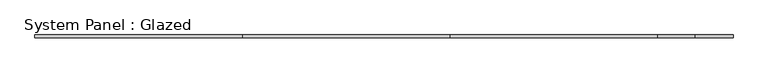
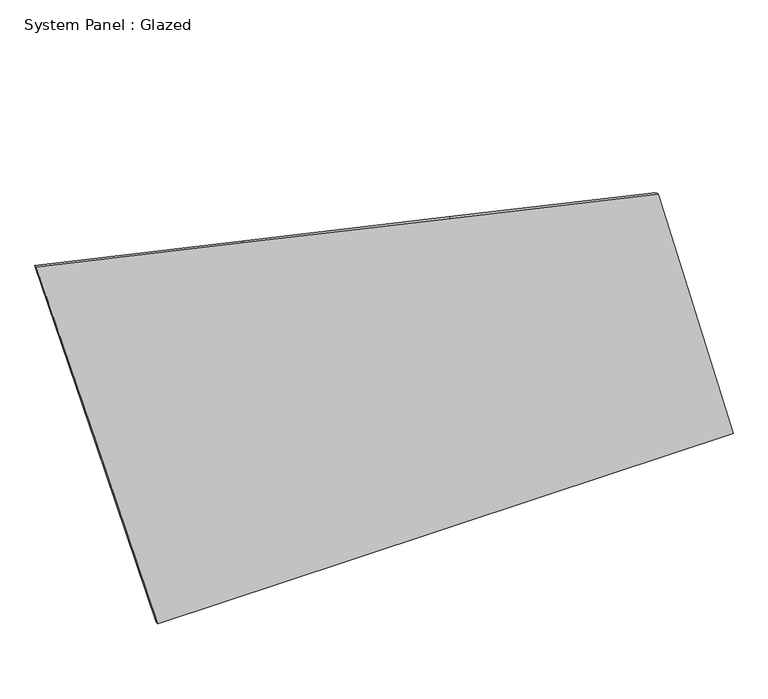
"""IFC4 building model written with IfcOpenShell, lengths in millimetres: plate geometry, System Panel : Glazed."""

from ifc_helpers import new_model, si_unit, frame, origin, place, context, project, spatial, polyline, outline, extrude, source, transform, mapped, element, save


def system_panel_glazed_187a64e4(model_context):
    return source(origin(), model_context, "Body", "SweptSolid", [
        extrude(outline(polyline([(0.0, -2112.1394868), (0.0, -327.8288499), (0.0, 1456.4817869), (0.0, 3240.7924238), (1300.2379466, 2891.490552), (2600.4758931, 2542.1886802), (3036.1291906, 614.5283122), (3471.7824882, -1313.1320558), (3907.4357857, -3240.7924238), (1953.7178929, -2676.4659553), (0.0, -2112.1394868)])), frame((0.0, -49.5, 0.0), z_axis=(0.0, 1.0, 0.0), x_axis=(0.0, 0.0, 1.0)), (0.0, 0.0, 1.0), 25.0),
    ])


if __name__ == "__main__":
    model = new_model("IFC4")
    model_context = context("Model", 3, world=origin())
    ifc_project = project(units=[si_unit("LENGTHUNIT", "METRE", prefix="MILLI")], contexts=[model_context])
    site = spatial("IfcSite", under=ifc_project)
    building = spatial("IfcBuilding", under=site)
    placement = place(None, origin())
    system_panel_glazed_shape = system_panel_glazed_187a64e4(model_context)
    element("IfcPlate", 1, ObjectType="System Panel : Glazed", at=placement, inside=building, context=model_context, shape_type="MappedRepresentation", body=[
        mapped(system_panel_glazed_shape, transform((0.0, 0.0, 0.0), x_axis=(1.0, 0.0, 0.0), y_axis=(0.0, 1.0, 0.0), z_axis=(0.0, 0.0, 1.0))),
    ])
    save(model, "model.ifc")

# Revit data of these elements
# Element 1 (IfcPlate, "System Panel : Glazed")
#   Materials on its faces: "Glass, Clear Glazing"
# Materials
#   "Glass, Clear Glazing": class "Glass", colour RGB 247 249 248, transparency 0.85, Description = "Clear glazing", Cost = 0
